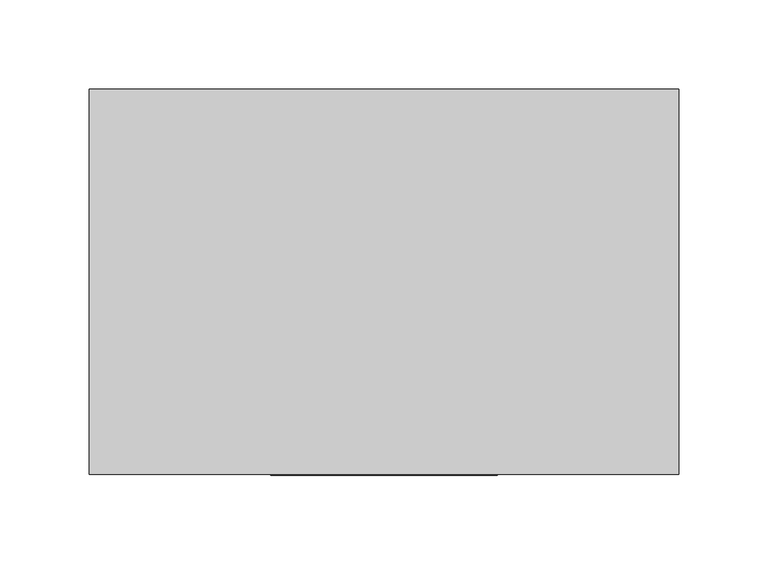
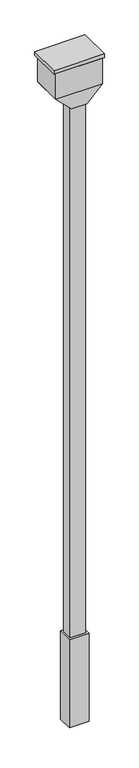
"""IFC4 building model written with IfcOpenShell, lengths in millimetres: proxy geometry, Wall Based Scupper & Leader Box with Downspout(boot) : Wall Based Scupper & Leader Box with Downspout."""

import ifcopenshell
import ifcopenshell.guid

model = None  # the IFC model being written
_history = None  # IfcOwnerHistory: only IFC2X3 demands one
_inside = {}  # id of a spatial element -> (the spatial element, [elements in it])
_under = {}  # id of a project, library or spatial element -> (it, [spatial elements below it])
_declared = {}  # id of a project -> (the project, [libraries it declares])
_typed = {}  # id of a type object -> (the type object, [elements of that type])
_made_of = {}  # id of a material, layer set ... -> (it, [elements and type objects made of it])


def new_model(schema):
    """Start an empty IFC model of exactly this schema.

    Asked for "IFC4X3", IfcOpenShell would pick the latest addendum, in which some entities
    have other attributes; the version numbers below select the first issue.
    IFC2X3 requires an IfcOwnerHistory on every rooted entity: one is made here for all.
    """
    global model, _history
    if schema == "IFC4X3":
        model = ifcopenshell.file(schema_version=(4, 3, 0, 0))
    else:
        model = ifcopenshell.file(schema=schema)
    _inside.clear()
    _under.clear()
    _declared.clear()
    _typed.clear()
    _made_of.clear()
    _history = None
    if model.schema == "IFC2X3":
        org = make("IfcOrganization", Name="unknown")
        user = make(
            "IfcPersonAndOrganization",
            ThePerson=make("IfcPerson", FamilyName="unknown"),
            TheOrganization=org,
        )
        app = make(
            "IfcApplication",
            ApplicationDeveloper=org,
            Version="unknown",
            ApplicationFullName="unknown",
            ApplicationIdentifier="unknown",
        )
        _history = make(
            "IfcOwnerHistory",
            OwningUser=user,
            OwningApplication=app,
            ChangeAction="ADDED",
            CreationDate=0,
        )
    return model


def make(cls, **values):
    """One entity of the class cls with the attributes given. An attribute that is None is left unset."""
    return model.create_entity(
        cls, **{name: value for name, value in values.items() if value is not None}
    )


def rooted(cls, **values):
    """An entity with a GlobalId (a new one), such as an element, a storey or a relation."""
    return make(cls, GlobalId=ifcopenshell.guid.new(), OwnerHistory=_history, **values)


def si_unit(unit_type, name, prefix=None):
    """IfcSIUnit, for example si_unit("LENGTHUNIT", "METRE", prefix="MILLI")."""
    return make("IfcSIUnit", UnitType=unit_type, Prefix=prefix, Name=name)


def assignment(units):
    """IfcUnitAssignment: the units of a project."""
    return None if units is None else make("IfcUnitAssignment", Units=units)


def point(xyz):
    """IfcCartesianPoint."""
    return None if xyz is None else make("IfcCartesianPoint", Coordinates=xyz)


def direction(xyz):
    """IfcDirection."""
    return None if xyz is None else make("IfcDirection", DirectionRatios=xyz)


def frame(location, z_axis=None, x_axis=None):
    """IfcAxis2Placement3D, a coordinate frame: its origin and axes. An axis left out is left unset."""
    return make(
        "IfcAxis2Placement3D",
        Location=point(location),
        Axis=direction(z_axis),
        RefDirection=direction(x_axis),
    )


def origin():
    """The frame at (0, 0, 0) with its axes left unset."""
    return frame((0.0, 0.0, 0.0))


def place(relative_to, where):
    """IfcLocalPlacement: puts the frame where relative to a parent placement (None: the world)."""
    return make(
        "IfcLocalPlacement", PlacementRelTo=relative_to, RelativePlacement=where
    )


def context(
    kind, dimensions, precision=None, world=None, true_north=None, identifier=None
):
    """IfcGeometricRepresentationContext, for example the 3D "Model" context."""
    return make(
        "IfcGeometricRepresentationContext",
        ContextIdentifier=identifier,
        ContextType=kind,
        CoordinateSpaceDimension=dimensions,
        Precision=precision,
        WorldCoordinateSystem=world,
        TrueNorth=true_north,
    )


def project(units=None, contexts=None):
    """IfcProject with its units and contexts."""
    return rooted(
        "IfcProject",
        Name="project",
        RepresentationContexts=contexts,
        UnitsInContext=assignment(units),
    )


def spatial(cls, under=None, at=None, **own):
    """A site, building, storey or space (cls), placed at a placement, below another one or the project."""
    s = rooted(cls, ObjectPlacement=at, **own)
    if under is not None:
        _under.setdefault(under.id(), (under, []))[1].append(s)
    return s


def polyline(points):
    """IfcPolyline through the points."""
    return make("IfcPolyline", Points=[point(p) for p in points])


def circle_curve(where, radius):
    """IfcCircle in the frame where."""
    return make("IfcCircle", Position=where, Radius=radius)


def outline(outer, holes=None, kind="AREA"):
    """IfcArbitraryClosedProfileDef: a profile drawn as a closed curve; with holes, ...WithVoids."""
    if holes is None:
        return make("IfcArbitraryClosedProfileDef", ProfileType=kind, OuterCurve=outer)
    return make(
        "IfcArbitraryProfileDefWithVoids",
        ProfileType=kind,
        OuterCurve=outer,
        InnerCurves=holes,
    )


def extrude(swept, where, along, depth):
    """IfcExtrudedAreaSolid: the profile swept, set in the frame where, extruded along a direction by depth."""
    return make(
        "IfcExtrudedAreaSolid",
        SweptArea=swept,
        Position=where,
        ExtrudedDirection=direction(along),
        Depth=depth,
    )


def faces_of(points, faces, orient=None, outer=None):
    """IfcFace entities. A face is a list of loops; a loop is a list of indices into points, from 0.

    orient and outer hold one flag for each loop. By default every Orientation is true, the
    first loop of a face is its IfcFaceOuterBound and the others are IfcFaceBound.
    """
    made = []
    for i, loops in enumerate(faces):
        bounds = []
        for j, loop in enumerate(loops):
            is_outer = j == 0 if outer is None else outer[i][j]
            bounds.append(
                make(
                    "IfcFaceOuterBound" if is_outer else "IfcFaceBound",
                    Bound=make("IfcPolyLoop", Polygon=[points[k] for k in loop]),
                    Orientation=True if orient is None else orient[i][j],
                )
            )
        made.append(make("IfcFace", Bounds=bounds))
    return made


def faceted_brep(points, faces, orient=None, outer=None, voids=None):
    """IfcFacetedBrep: a solid bounded by flat faces; with voids (closed shells), ...WithVoids."""
    shared = [point(p) for p in points]
    hull = make("IfcClosedShell", CfsFaces=faces_of(shared, faces, orient, outer))
    if voids is None:
        return make("IfcFacetedBrep", Outer=hull)
    return make(
        "IfcFacetedBrepWithVoids",
        Outer=hull,
        Voids=[
            make(cls, CfsFaces=faces_of(shared, fs, o, b)) for cls, fs, o, b in voids
        ],
    )


def shape(context_of_items, identifier, shape_type, items):
    """IfcShapeRepresentation: the items that make up one representation, for example the "Body"."""
    return make(
        "IfcShapeRepresentation",
        ContextOfItems=context_of_items,
        RepresentationIdentifier=identifier,
        RepresentationType=shape_type,
        Items=items,
    )


def source(mapping_origin, context_of_items, identifier, shape_type, items):
    """IfcRepresentationMap: a shape defined once, which mapped items show again and again."""
    return make(
        "IfcRepresentationMap",
        MappingOrigin=mapping_origin,
        MappedRepresentation=shape(context_of_items, identifier, shape_type, items),
    )


def transform(
    local_origin,
    x_axis=None,
    y_axis=None,
    z_axis=None,
    scale=None,
    scale2=None,
    scale3=None,
    uniform=True,
):
    """IfcCartesianTransformationOperator3D, or its non-uniform kind. x_axis, y_axis, z_axis: its Axis1, 2, 3."""
    if uniform:
        return make(
            "IfcCartesianTransformationOperator3D",
            Axis1=direction(x_axis),
            Axis2=direction(y_axis),
            LocalOrigin=point(local_origin),
            Scale=scale,
            Axis3=direction(z_axis),
        )
    return make(
        "IfcCartesianTransformationOperator3DnonUniform",
        Axis1=direction(x_axis),
        Axis2=direction(y_axis),
        LocalOrigin=point(local_origin),
        Scale=scale,
        Axis3=direction(z_axis),
        Scale2=scale2,
        Scale3=scale3,
    )


def mapped(mapping_source, mapping_target):
    """IfcMappedItem: shows the shape of a source again, moved by a transform."""
    return make(
        "IfcMappedItem", MappingSource=mapping_source, MappingTarget=mapping_target
    )


def made_of(thing, what):
    """Note that an element or type object is made of a material, layer set ...; save() writes the relation."""
    if what is not None:
        _made_of.setdefault(what.id(), (what, []))[1].append(thing)
    return thing


def element(
    cls,
    number,
    at=None,
    inside=None,
    cuts=None,
    type_object=None,
    material=None,
    context=None,
    identifier="Body",
    shape_type=None,
    held_by="IfcProductDefinitionShape",
    body=None,
    shapes=None,
    **own,
):
    """One element of the class cls, such as IfcWall. Its Tag is "e" and its number.

    at: its placement. inside: the storey or other place that contains it. cuts: it is an
    opening in that element (IfcRelVoidsElement). A single representation is given by context,
    identifier, shape_type and body (its items); several are given by shapes. held_by: the class
    of the entity that holds the representations. save() writes the other relations.
    """
    e = rooted(cls, Tag="e%d" % number, ObjectPlacement=at, **own)
    if body is not None:
        shapes = [shape(context, identifier, shape_type, body)]
    if shapes is not None:
        e.Representation = make(held_by, Representations=shapes)
    if inside is not None:
        _inside.setdefault(inside.id(), (inside, []))[1].append(e)
    if cuts is not None:
        rooted(
            "IfcRelVoidsElement", RelatingBuildingElement=cuts, RelatedOpeningElement=e
        )
    if type_object is not None:
        _typed.setdefault(type_object.id(), (type_object, []))[1].append(e)
    return made_of(e, material)


def aggregate(whole, parts):
    """IfcRelAggregates: a whole, such as a stair, and the parts it consists of."""
    return rooted("IfcRelAggregates", RelatingObject=whole, RelatedObjects=parts)


def save(model, path):
    """Write the relations noted so far, then the file.

    IfcRelAggregates (storeys below a building ...), IfcRelContainedInSpatialStructure (elements
    in a storey), IfcRelDefinesByType, IfcRelAssociatesMaterial and IfcRelDeclares: one each for
    every whole, place, type object, material and project.
    """
    for whole, parts in _under.values():
        aggregate(whole, parts)
    for where, things in _inside.values():
        rooted(
            "IfcRelContainedInSpatialStructure",
            RelatedElements=things,
            RelatingStructure=where,
        )
    for kind, things in _typed.values():
        rooted("IfcRelDefinesByType", RelatedObjects=things, RelatingType=kind)
    for what, things in _made_of.values():
        rooted("IfcRelAssociatesMaterial", RelatedObjects=things, RelatingMaterial=what)
    for by, libraries in _declared.values():
        rooted("IfcRelDeclares", RelatingContext=by, RelatedDefinitions=libraries)
    model.write(path)


def plane_surface(at):
    """IfcPlane: the flat surface through the origin of the frame at, square to its z axis."""
    return make("IfcPlane", Position=at)


def revolved_surface(curve, axis_point, axis_direction):
    """IfcSurfaceOfRevolution: the curve turned about the line through axis_point along axis_direction."""
    return make(
        "IfcSurfaceOfRevolution",
        SweptCurve=make("IfcArbitraryOpenProfileDef", ProfileType="CURVE", Curve=curve),
        AxisPosition=make("IfcAxis1Placement", Location=point(axis_point), Axis=direction(axis_direction)),
    )


def advanced_brep(points, edges, surfaces, faces):
    """IfcAdvancedBrep: a solid bounded by faces that lie on surfaces and meet in shared edges.

    An edge is (start, end): straight between two places in points (the first is 0);
    or (start, end, curve); or (start, end, curve, False) where it runs against its curve.
    A face is (place in surfaces, loops), or (place, loops, False) where it looks against
    its surface's normal. A loop lists edges by number (the first is 1), with a minus sign
    where the edge is run from its end to its start. The first loop is the outer one.
    """
    corners = [point(p) for p in points]
    vertices = [make("IfcVertexPoint", VertexGeometry=c) for c in corners]
    made = []
    for start, end, *more in edges:
        made.append(
            make(
                "IfcEdgeCurve",
                EdgeStart=vertices[start],
                EdgeEnd=vertices[end],
                EdgeGeometry=more[0] if more else make("IfcPolyline", Points=[corners[start], corners[end]]),
                SameSense=more[1] if len(more) > 1 else True,
            )
        )
    hull = []
    for where, loops, *sense in faces:
        bounds = []
        for j, loop in enumerate(loops):
            ring = [make("IfcOrientedEdge", EdgeElement=made[abs(k) - 1], Orientation=k > 0) for k in loop]
            bounds.append(
                make(
                    "IfcFaceOuterBound" if j == 0 else "IfcFaceBound",
                    Bound=make("IfcEdgeLoop", EdgeList=ring),
                    Orientation=True,
                )
            )
        hull.append(make("IfcAdvancedFace", Bounds=bounds, FaceSurface=surfaces[where], SameSense=sense[0] if sense else True))
    return make("IfcAdvancedBrep", Outer=make("IfcClosedShell", CfsFaces=hull))


def generic_models_870a4fbb(model_context):
    return source(origin(), model_context, "Body", "SolidModel", [
        faceted_brep([(70.7824157, 215.9, -3841.75), (-56.2175843, 215.9, -3841.75), (-56.2175843, 114.3, -3841.75), (70.7824157, 114.3, -3841.75), (58.0824157, 127.0, -3841.75), (-43.5175843, 127.0, -3841.75), (-43.5175843, 203.2, -3841.75), (58.0824157, 203.2, -3841.75), (70.7824157, 215.9, -4451.35), (70.7824157, 114.3, -4451.35), (-56.2175843, 114.3, -4451.35), (-56.2175843, 215.9, -4451.35), (-43.5175843, 127.0, -184.15), (58.0824157, 127.0, -184.15), (58.0824157, 203.2, -184.15), (-43.5175843, 203.2, -184.15)], [[[0, 1, 2, 3], [4, 5, 6, 7]], [[8, 9, 10, 11]], [[1, 0, 8, 11]], [[2, 1, 11, 10]], [[3, 2, 10, 9]], [[0, 3, 9, 8]], [[12, 13, 14, 15]], [[13, 12, 5, 4]], [[14, 13, 4, 7]], [[15, 14, 7, 6]], [[12, 15, 6, 5]]]),
        advanced_brep(
        [(159.6824157, 114.3, -82.55), (159.6824157, 114.3, 95.25), (-145.1175843, 114.3, 95.25), (-145.1175843, 114.3, -82.55), (159.6824157, 317.5, -82.55), (-145.1175843, 317.5, -82.55), (-145.1175843, 317.5, 95.25), (159.6824157, 317.5, 95.25), (-11.7675843, 317.5, 46.7708134), (26.3324157, 317.5, 46.7708134), (-11.7675843, 307.693698, 46.7708134), (26.3324157, 307.693698, 46.7708134)],
        [
            (0, 1),
            (1, 2),
            (2, 3),
            (3, 0),
            (4, 5),
            (5, 6),
            (6, 7),
            (7, 4),
            (8, 9, circle_curve(frame((7.2824157, 317.5, 46.7708134), z_axis=(0.0, -1.0, 0.0), x_axis=(1.0, 0.0, 0.0)), 19.05)),
            (9, 8, circle_curve(frame((7.2824157, 317.5, 46.7708134), z_axis=(0.0, -1.0, 0.0), x_axis=(1.0, 0.0, 0.0)), 19.05)),
            (0, 4),
            (7, 1),
            (6, 2),
            (5, 3),
            (10, 11, circle_curve(frame((7.2824157, 307.693698, 46.7708134), z_axis=(0.0, 1.0, 0.0), x_axis=(1.0, 0.0, 0.0)), 19.05)),
            (11, 10, circle_curve(frame((7.2824157, 307.693698, 46.7708134), z_axis=(0.0, 1.0, 0.0), x_axis=(1.0, 0.0, 0.0)), 19.05)),
            (11, 9),
            (8, 10),
        ],
        [
            plane_surface(frame((159.6824157, 114.3, 95.25), z_axis=(0.0, -1.0, 0.0), x_axis=(0.0, 0.0, 1.0))),
            plane_surface(frame((159.6824157, 317.5, 95.25), z_axis=(0.0, 1.0, 0.0), x_axis=(0.0, 0.0, -1.0))),
            plane_surface(frame((159.6824157, 114.3, -82.55), z_axis=(1.0, 0.0, 0.0), x_axis=(0.0, 1.0, 0.0))),
            plane_surface(frame((159.6824157, 114.3, 95.25), z_axis=(0.0, 0.0, 1.0), x_axis=(0.0, 1.0, 0.0))),
            plane_surface(frame((-145.1175843, 114.3, 95.25), z_axis=(-1.0, 0.0, 0.0), x_axis=(0.0, 1.0, 0.0))),
            plane_surface(frame((-145.1175843, 114.3, -82.55), z_axis=(0.0, 0.0, -1.0), x_axis=(0.0, 1.0, 0.0))),
            plane_surface(frame((26.3324157, 307.693698, 46.7708134), z_axis=(0.0, 1.0, 0.0), x_axis=(0.0, 0.0, 1.0))),
            revolved_surface(polyline([(26.3324157, 307.693698, 46.7708134), (26.3324157, 317.5, 46.7708134)]), (7.2824157, 358.1283044, 46.7708134), (0.0, -1.0, 0.0)),
        ],
        [
            (0, [[1, 2, 3, 4]]),
            (1, [[5, 6, 7, 8], [9, 10]]),
            (2, [[-1, 11, -8, 12]]),
            (3, [[-2, -12, -7, 13]]),
            (4, [[-3, -13, -6, 14]]),
            (5, [[-4, -14, -5, -11]]),
            (6, [[15, 16]]),
            (7, [[-16, 17, -9, 18]]),
            (7, [[-15, -18, -10, -17]]),
        ],
    ),
        faceted_brep([(-145.1175843, 114.3, -82.55), (159.6824157, 114.3, -82.55), (159.6824157, 317.5, -82.55), (-145.1175843, 317.5, -82.55), (-43.5175843, 114.3, -184.15), (-43.5175843, 215.9, -184.15), (58.0824157, 215.9, -184.15), (58.0824157, 114.3, -184.15)], [[[0, 1, 2, 3]], [[4, 5, 6, 7]], [[4, 7, 1, 0]], [[7, 6, 2, 1]], [[6, 5, 3, 2]], [[5, 4, 0, 3]]]),
        extrude(outline(polyline([(172.3824157, 114.3), (-157.8175843, 114.3), (-157.8175843, 330.2), (172.3824157, 330.2), (172.3824157, 114.3)])), frame((0.0, 0.0, 95.25), z_axis=(0.0, 0.0, 1.0), x_axis=(1.0, 0.0, 0.0)), (0.0, 0.0, 1.0), 25.4),
    ])


if __name__ == "__main__":
    model = new_model("IFC4")
    model_context = context("Model", 3, world=origin())
    ifc_project = project(units=[si_unit("LENGTHUNIT", "METRE", prefix="MILLI")], contexts=[model_context])
    site = spatial("IfcSite", under=ifc_project)
    building = spatial("IfcBuilding", under=site)
    placement = place(None, origin())
    generic_models_shape = generic_models_870a4fbb(model_context)
    element("IfcBuildingElementProxy", 1, Name="Wall Based Scupper & Leader Box with Downspout(boot) : Wall Based Scupper & Leader Box with Downspout", ObjectType="Wall Based Scupper & Leader Box with Downspout(boot) : Wall Based Scupper & Leader Box with Downspout", at=placement, inside=building, context=model_context, shape_type="MappedRepresentation", body=[
        mapped(generic_models_shape, transform((0.0, 0.0, 0.0), x_axis=(1.0, 0.0, 0.0), y_axis=(0.0, 1.0, 0.0), z_axis=(0.0, 0.0, 1.0))),
    ])
    save(model, "model.ifc")

# Revit data of these elements
# Type "Wall Based Scupper & Leader Box with Downspout(boot) : Wall Based Scupper & Leader Box with Downspout"
#   Keynote = "07710.B4"
#   boot height [instance default] = 2' - 0"
#   Width Between Box & Wall = 0' - 0 1/2"
#   Scupper Width = 0' - 5 1/2"
#   Scupper Height = 0' - 3 1/2"
#   Leader Box Lid Width = 1' - 1"
#   Leader Box Lid Depth = 0' - 8 1/2"
#   Downspout Width = 0' - 4"
#   Downspout Height [instance default] = 12' - 0"
#   Downspout Depth = 0' - 3"
#   Box Width 01 = 1' - 0"
#   Box Void Width = 0' - 11 1/2"
#   Box Void Depth = 0' - 7 1/2"
#   Box Height 02 = 0' - 4"
#   Box Height 01 = 0' - 7"
#   Box Depth 01 = 0' - 8"
#   Boot = no
#   Default Elevation = 0
#   Assembly Code = ""
# Element 1 (IfcBuildingElementProxy, "Wall Based Scupper & Leader Box with Downspout(boot) : Wall Based Scupper & Leader Box with Downspout")
#   Downspout Height = 14' - 0"
#   Materials on its faces: "Default"
# Materials
#   "Default": class "Miscellaneous", colour RGB 127 127 127, transparency 0
